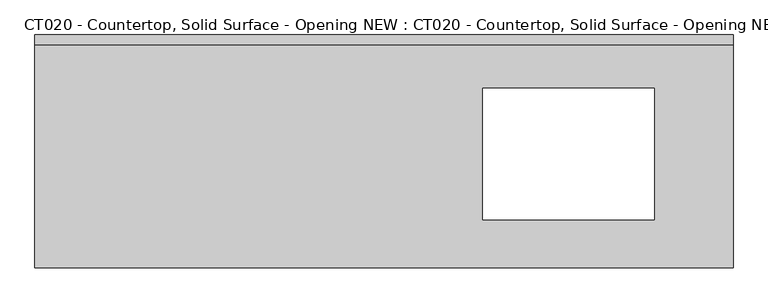
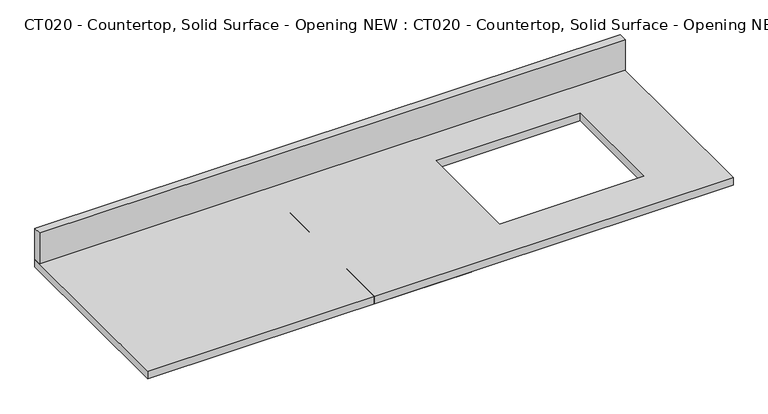
"""IFC4 building model written with IfcOpenShell, lengths in millimetres: proxy geometry, CT020 - Countertop, Solid Surface - Opening NEW : CT020 - Countertop, Solid Surface - Opening NEW."""

import ifcopenshell
import ifcopenshell.guid

model = None  # the IFC model being written
_history = None  # IfcOwnerHistory: only IFC2X3 demands one
_inside = {}  # id of a spatial element -> (the spatial element, [elements in it])
_under = {}  # id of a project, library or spatial element -> (it, [spatial elements below it])
_declared = {}  # id of a project -> (the project, [libraries it declares])
_typed = {}  # id of a type object -> (the type object, [elements of that type])
_made_of = {}  # id of a material, layer set ... -> (it, [elements and type objects made of it])


def new_model(schema):
    """Start an empty IFC model of exactly this schema.

    Asked for "IFC4X3", IfcOpenShell would pick the latest addendum, in which some entities
    have other attributes; the version numbers below select the first issue.
    IFC2X3 requires an IfcOwnerHistory on every rooted entity: one is made here for all.
    """
    global model, _history
    if schema == "IFC4X3":
        model = ifcopenshell.file(schema_version=(4, 3, 0, 0))
    else:
        model = ifcopenshell.file(schema=schema)
    _inside.clear()
    _under.clear()
    _declared.clear()
    _typed.clear()
    _made_of.clear()
    _history = None
    if model.schema == "IFC2X3":
        org = make("IfcOrganization", Name="unknown")
        user = make(
            "IfcPersonAndOrganization",
            ThePerson=make("IfcPerson", FamilyName="unknown"),
            TheOrganization=org,
        )
        app = make(
            "IfcApplication",
            ApplicationDeveloper=org,
            Version="unknown",
            ApplicationFullName="unknown",
            ApplicationIdentifier="unknown",
        )
        _history = make(
            "IfcOwnerHistory",
            OwningUser=user,
            OwningApplication=app,
            ChangeAction="ADDED",
            CreationDate=0,
        )
    return model


def make(cls, **values):
    """One entity of the class cls with the attributes given. An attribute that is None is left unset."""
    return model.create_entity(
        cls, **{name: value for name, value in values.items() if value is not None}
    )


def rooted(cls, **values):
    """An entity with a GlobalId (a new one), such as an element, a storey or a relation."""
    return make(cls, GlobalId=ifcopenshell.guid.new(), OwnerHistory=_history, **values)


def si_unit(unit_type, name, prefix=None):
    """IfcSIUnit, for example si_unit("LENGTHUNIT", "METRE", prefix="MILLI")."""
    return make("IfcSIUnit", UnitType=unit_type, Prefix=prefix, Name=name)


def assignment(units):
    """IfcUnitAssignment: the units of a project."""
    return None if units is None else make("IfcUnitAssignment", Units=units)


def point(xyz):
    """IfcCartesianPoint."""
    return None if xyz is None else make("IfcCartesianPoint", Coordinates=xyz)


def direction(xyz):
    """IfcDirection."""
    return None if xyz is None else make("IfcDirection", DirectionRatios=xyz)


def frame(location, z_axis=None, x_axis=None):
    """IfcAxis2Placement3D, a coordinate frame: its origin and axes. An axis left out is left unset."""
    return make(
        "IfcAxis2Placement3D",
        Location=point(location),
        Axis=direction(z_axis),
        RefDirection=direction(x_axis),
    )


def origin():
    """The frame at (0, 0, 0) with its axes left unset."""
    return frame((0.0, 0.0, 0.0))


def origin_with_axes():
    """The frame at (0, 0, 0) with the z axis (0, 0, 1) and the x axis (1, 0, 0) written out."""
    return frame((0.0, 0.0, 0.0), z_axis=(0.0, 0.0, 1.0), x_axis=(1.0, 0.0, 0.0))


def place(relative_to, where):
    """IfcLocalPlacement: puts the frame where relative to a parent placement (None: the world)."""
    return make(
        "IfcLocalPlacement", PlacementRelTo=relative_to, RelativePlacement=where
    )


def context(
    kind, dimensions, precision=None, world=None, true_north=None, identifier=None
):
    """IfcGeometricRepresentationContext, for example the 3D "Model" context."""
    return make(
        "IfcGeometricRepresentationContext",
        ContextIdentifier=identifier,
        ContextType=kind,
        CoordinateSpaceDimension=dimensions,
        Precision=precision,
        WorldCoordinateSystem=world,
        TrueNorth=true_north,
    )


def project(units=None, contexts=None):
    """IfcProject with its units and contexts."""
    return rooted(
        "IfcProject",
        Name="project",
        RepresentationContexts=contexts,
        UnitsInContext=assignment(units),
    )


def spatial(cls, under=None, at=None, **own):
    """A site, building, storey or space (cls), placed at a placement, below another one or the project."""
    s = rooted(cls, ObjectPlacement=at, **own)
    if under is not None:
        _under.setdefault(under.id(), (under, []))[1].append(s)
    return s


def polyline(points):
    """IfcPolyline through the points."""
    return make("IfcPolyline", Points=[point(p) for p in points])


def outline(outer, holes=None, kind="AREA"):
    """IfcArbitraryClosedProfileDef: a profile drawn as a closed curve; with holes, ...WithVoids."""
    if holes is None:
        return make("IfcArbitraryClosedProfileDef", ProfileType=kind, OuterCurve=outer)
    return make(
        "IfcArbitraryProfileDefWithVoids",
        ProfileType=kind,
        OuterCurve=outer,
        InnerCurves=holes,
    )


def extrude(swept, where, along, depth):
    """IfcExtrudedAreaSolid: the profile swept, set in the frame where, extruded along a direction by depth."""
    return make(
        "IfcExtrudedAreaSolid",
        SweptArea=swept,
        Position=where,
        ExtrudedDirection=direction(along),
        Depth=depth,
    )


def shape(context_of_items, identifier, shape_type, items):
    """IfcShapeRepresentation: the items that make up one representation, for example the "Body"."""
    return make(
        "IfcShapeRepresentation",
        ContextOfItems=context_of_items,
        RepresentationIdentifier=identifier,
        RepresentationType=shape_type,
        Items=items,
    )


def source(mapping_origin, context_of_items, identifier, shape_type, items):
    """IfcRepresentationMap: a shape defined once, which mapped items show again and again."""
    return make(
        "IfcRepresentationMap",
        MappingOrigin=mapping_origin,
        MappedRepresentation=shape(context_of_items, identifier, shape_type, items),
    )


def transform(
    local_origin,
    x_axis=None,
    y_axis=None,
    z_axis=None,
    scale=None,
    scale2=None,
    scale3=None,
    uniform=True,
):
    """IfcCartesianTransformationOperator3D, or its non-uniform kind. x_axis, y_axis, z_axis: its Axis1, 2, 3."""
    if uniform:
        return make(
            "IfcCartesianTransformationOperator3D",
            Axis1=direction(x_axis),
            Axis2=direction(y_axis),
            LocalOrigin=point(local_origin),
            Scale=scale,
            Axis3=direction(z_axis),
        )
    return make(
        "IfcCartesianTransformationOperator3DnonUniform",
        Axis1=direction(x_axis),
        Axis2=direction(y_axis),
        LocalOrigin=point(local_origin),
        Scale=scale,
        Axis3=direction(z_axis),
        Scale2=scale2,
        Scale3=scale3,
    )


def mapped(mapping_source, mapping_target):
    """IfcMappedItem: shows the shape of a source again, moved by a transform."""
    return make(
        "IfcMappedItem", MappingSource=mapping_source, MappingTarget=mapping_target
    )


def made_of(thing, what):
    """Note that an element or type object is made of a material, layer set ...; save() writes the relation."""
    if what is not None:
        _made_of.setdefault(what.id(), (what, []))[1].append(thing)
    return thing


def element(
    cls,
    number,
    at=None,
    inside=None,
    cuts=None,
    type_object=None,
    material=None,
    context=None,
    identifier="Body",
    shape_type=None,
    held_by="IfcProductDefinitionShape",
    body=None,
    shapes=None,
    **own,
):
    """One element of the class cls, such as IfcWall. Its Tag is "e" and its number.

    at: its placement. inside: the storey or other place that contains it. cuts: it is an
    opening in that element (IfcRelVoidsElement). A single representation is given by context,
    identifier, shape_type and body (its items); several are given by shapes. held_by: the class
    of the entity that holds the representations. save() writes the other relations.
    """
    e = rooted(cls, Tag="e%d" % number, ObjectPlacement=at, **own)
    if body is not None:
        shapes = [shape(context, identifier, shape_type, body)]
    if shapes is not None:
        e.Representation = make(held_by, Representations=shapes)
    if inside is not None:
        _inside.setdefault(inside.id(), (inside, []))[1].append(e)
    if cuts is not None:
        rooted(
            "IfcRelVoidsElement", RelatingBuildingElement=cuts, RelatedOpeningElement=e
        )
    if type_object is not None:
        _typed.setdefault(type_object.id(), (type_object, []))[1].append(e)
    return made_of(e, material)


def aggregate(whole, parts):
    """IfcRelAggregates: a whole, such as a stair, and the parts it consists of."""
    return rooted("IfcRelAggregates", RelatingObject=whole, RelatedObjects=parts)


def save(model, path):
    """Write the relations noted so far, then the file.

    IfcRelAggregates (storeys below a building ...), IfcRelContainedInSpatialStructure (elements
    in a storey), IfcRelDefinesByType, IfcRelAssociatesMaterial and IfcRelDeclares: one each for
    every whole, place, type object, material and project.
    """
    for whole, parts in _under.values():
        aggregate(whole, parts)
    for where, things in _inside.values():
        rooted(
            "IfcRelContainedInSpatialStructure",
            RelatedElements=things,
            RelatingStructure=where,
        )
    for kind, things in _typed.values():
        rooted("IfcRelDefinesByType", RelatedObjects=things, RelatingType=kind)
    for what, things in _made_of.values():
        rooted("IfcRelAssociatesMaterial", RelatedObjects=things, RelatingMaterial=what)
    for by, libraries in _declared.values():
        rooted("IfcRelDeclares", RelatingContext=by, RelatedDefinitions=libraries)
    model.write(path)


def ct020_countertop_solid_surface_opening_new_ct020_countertop_3a9c1b0d(model_context):
    return source(origin(), model_context, "Body", "SweptSolid", [
        extrude(outline(polyline([(968.1059067, 304.8), (968.1059067, -304.8), (-858.5795225, -304.8), (-858.5795225, 304.8), (968.1059067, 304.8)]), holes=[polyline([(762.0, 165.1), (313.1178879, 165.1), (313.1178879, -178.386638), (762.0, -178.386638), (762.0, 165.1)])]), origin_with_axes(), (0.0, 0.0, 1.0), 25.4),
        extrude(outline(polyline([(-858.5795225, 279.4), (-858.5795225, 304.8), (968.1059067, 304.8), (968.1059067, 279.4), (-858.5795225, 279.4)])), frame((0.0, 0.0, 25.4), z_axis=(0.0, 0.0, 1.0), x_axis=(1.0, 0.0, 0.0)), (0.0, 0.0, 1.0), 101.6),
        extrude(outline(polyline([(-152.4, 304.8), (152.4, 304.8), (152.4, -304.8), (-152.4, -304.8), (-152.4, 0.0), (-152.4, 304.8)])), origin_with_axes(), (0.0, 0.0, 1.0), 25.4),
    ])


if __name__ == "__main__":
    model = new_model("IFC4")
    model_context = context("Model", 3, world=origin())
    ifc_project = project(units=[si_unit("LENGTHUNIT", "METRE", prefix="MILLI")], contexts=[model_context])
    site = spatial("IfcSite", under=ifc_project)
    building = spatial("IfcBuilding", under=site)
    placement = place(None, origin())
    ct020_countertop_solid_surface_opening_new_ct020_countertop_shape = ct020_countertop_solid_surface_opening_new_ct020_countertop_3a9c1b0d(model_context)
    element("IfcBuildingElementProxy", 1, Name="CT020 - Countertop, Solid Surface - Opening NEW : CT020 - Countertop, Solid Surface - Opening NEW", ObjectType="CT020 - Countertop, Solid Surface - Opening NEW : CT020 - Countertop, Solid Surface - Opening NEW", at=placement, inside=building, context=model_context, shape_type="MappedRepresentation", body=[
        mapped(ct020_countertop_solid_surface_opening_new_ct020_countertop_shape, transform((0.0, 0.0, 0.0), x_axis=(1.0, 0.0, 0.0), y_axis=(0.0, 1.0, 0.0), z_axis=(0.0, 0.0, 1.0))),
    ])
    save(model, "model.ifc")

# Revit data of these elements
# Type "CT020 - Countertop, Solid Surface - Opening NEW : CT020 - Countertop, Solid Surface - Opening NEW"
#   Watts2 = "0"
#   Watts1 = "0"
#   Unit_Issue = "LF"
#   UTIL_6_Misc = "-"
#   UTIL_5_NonMedGas = "-"
#   UTIL_4_MiscGas = "-"
#   UTIL_3_MedGas = "-"
#   UTIL_2_Elec = "-"
#   UTIL_1_WaterDrain = "-"
#   Nomenclature = "Countertop, Solid Surface"
#   NSN = "6530"
#   Location [instance default] = ""
#   JSN = "CT020"
#   Fund_Source_VA = "-"
#   Fund_Source_Navy = "-"
#   Fund_Source_Army = "-"
#   Fund_Source_AF = "-"
#   ELEC_Volts2 = "0"
#   ELEC_Volts1 = "0"
#   ELEC_Phase2 = "0"
#   ELEC_Phase1 = "0"
#   ELEC_HertzSwitch = "0"
#   ELEC_HertzDependent = "0"
#   ELEC_Hertz = "0"
#   ELEC_Amps2 = "0"
#   ELEC_Amps1 = "0"
#   DetailDescription = "High pressure laminate countertop (composition of wood particle core with plastic laminate surface) having a hard smooth surface finish, standard thickness of 1\", and a 4\" butt backsplash/curb. Also referred to as a work surface or work top. Available in a wide choice of colors, patterns, and depths. Used in general purpose areas requiring a basic work surface arrangement with limited heat resistance and poor chemical resistance. Pricing based upon a 24\" depth."
#   CAT_VA = "A"
#   CAT_Navy = "A"
#   CAT_IHS = "-"
#   CAT_Army = "A"
#   CAT_AF = "A"
#   BTUperhour = "0"
#   Weight_IP = 14
#   OpeningLength2 [instance default] = 1' - 6"
#   OpeningLength [instance default] = 3' - 2"
#   OpeningDepth2 [instance default] = 0' - 8"
#   OpeningDepth [instance default] = 0' - 8"
#   DIM_Width_IP = 1' - 0"
#   DIM_Height_IP = 0' - 1"
#   DIM_Depth_IP = 2' - 0"
#   CustomLength2 [instance default] = 3' - 0"
#   CustomLength [instance default] = 3' - 0"
#   Assembly Code = ""
# Element 1 (IfcBuildingElementProxy, "CT020 - Countertop, Solid Surface - Opening NEW : CT020 - Countertop, Solid Surface - Opening NEW")
#   OpeningLength2 = 0' - 4.78874"
#   OpeningLength = 1' - 0.88378"
#   OpeningDepth2 = 0' - 6 1/2"
#   OpeningDepth = 0' - 7.0231"
#   CustomLength2 = 3' - 2.11441"
#   CustomLength = 2' - 9.80234"
#   Materials on its faces: "CounterTopFinish", "EquipSpace"
# Materials
#   "CounterTopFinish": class "Unassigned", colour RGB 139 121 96, transparency 0
#   "EquipSpace": class "Unassigned", colour RGB 221 217 195, transparency 0.5
